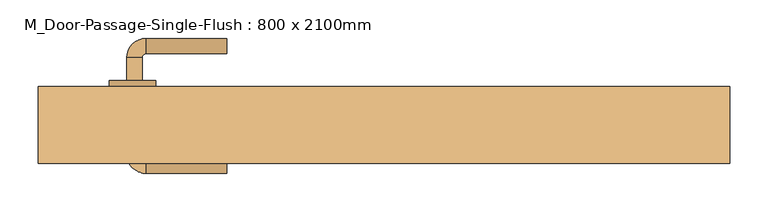
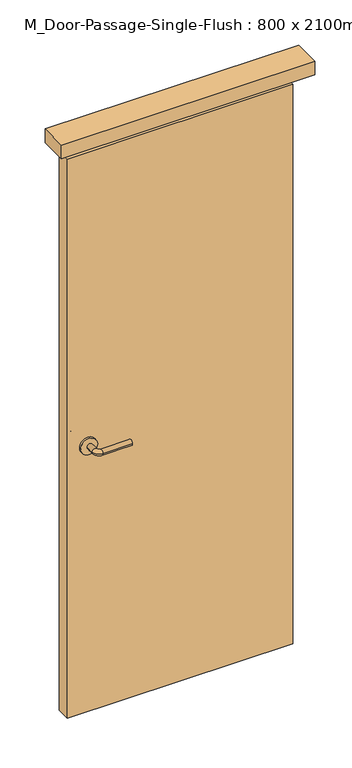
"""IFC4 building model written with IfcOpenShell, lengths in millimetres: door geometry, M_Door-Passage-Single-Flush : 800 x 2100mm."""

import ifcopenshell
import ifcopenshell.guid

model = None  # the IFC model being written
_history = None  # IfcOwnerHistory: only IFC2X3 demands one
_inside = {}  # id of a spatial element -> (the spatial element, [elements in it])
_under = {}  # id of a project, library or spatial element -> (it, [spatial elements below it])
_declared = {}  # id of a project -> (the project, [libraries it declares])
_typed = {}  # id of a type object -> (the type object, [elements of that type])
_made_of = {}  # id of a material, layer set ... -> (it, [elements and type objects made of it])


def new_model(schema):
    """Start an empty IFC model of exactly this schema.

    Asked for "IFC4X3", IfcOpenShell would pick the latest addendum, in which some entities
    have other attributes; the version numbers below select the first issue.
    IFC2X3 requires an IfcOwnerHistory on every rooted entity: one is made here for all.
    """
    global model, _history
    if schema == "IFC4X3":
        model = ifcopenshell.file(schema_version=(4, 3, 0, 0))
    else:
        model = ifcopenshell.file(schema=schema)
    _inside.clear()
    _under.clear()
    _declared.clear()
    _typed.clear()
    _made_of.clear()
    _history = None
    if model.schema == "IFC2X3":
        org = make("IfcOrganization", Name="unknown")
        user = make(
            "IfcPersonAndOrganization",
            ThePerson=make("IfcPerson", FamilyName="unknown"),
            TheOrganization=org,
        )
        app = make(
            "IfcApplication",
            ApplicationDeveloper=org,
            Version="unknown",
            ApplicationFullName="unknown",
            ApplicationIdentifier="unknown",
        )
        _history = make(
            "IfcOwnerHistory",
            OwningUser=user,
            OwningApplication=app,
            ChangeAction="ADDED",
            CreationDate=0,
        )
    return model


def make(cls, **values):
    """One entity of the class cls with the attributes given. An attribute that is None is left unset."""
    return model.create_entity(
        cls, **{name: value for name, value in values.items() if value is not None}
    )


def rooted(cls, **values):
    """An entity with a GlobalId (a new one), such as an element, a storey or a relation."""
    return make(cls, GlobalId=ifcopenshell.guid.new(), OwnerHistory=_history, **values)


def si_unit(unit_type, name, prefix=None):
    """IfcSIUnit, for example si_unit("LENGTHUNIT", "METRE", prefix="MILLI")."""
    return make("IfcSIUnit", UnitType=unit_type, Prefix=prefix, Name=name)


def assignment(units):
    """IfcUnitAssignment: the units of a project."""
    return None if units is None else make("IfcUnitAssignment", Units=units)


def point(xyz):
    """IfcCartesianPoint."""
    return None if xyz is None else make("IfcCartesianPoint", Coordinates=xyz)


def direction(xyz):
    """IfcDirection."""
    return None if xyz is None else make("IfcDirection", DirectionRatios=xyz)


def frame(location, z_axis=None, x_axis=None):
    """IfcAxis2Placement3D, a coordinate frame: its origin and axes. An axis left out is left unset."""
    return make(
        "IfcAxis2Placement3D",
        Location=point(location),
        Axis=direction(z_axis),
        RefDirection=direction(x_axis),
    )


def frame_2d(location, x_axis=None):
    """IfcAxis2Placement2D, a coordinate frame in the plane: its origin and x axis."""
    return make(
        "IfcAxis2Placement2D", Location=point(location), RefDirection=direction(x_axis)
    )


def origin():
    """The frame at (0, 0, 0) with its axes left unset."""
    return frame((0.0, 0.0, 0.0))


def origin_with_axes():
    """The frame at (0, 0, 0) with the z axis (0, 0, 1) and the x axis (1, 0, 0) written out."""
    return frame((0.0, 0.0, 0.0), z_axis=(0.0, 0.0, 1.0), x_axis=(1.0, 0.0, 0.0))


def place(relative_to, where):
    """IfcLocalPlacement: puts the frame where relative to a parent placement (None: the world)."""
    return make(
        "IfcLocalPlacement", PlacementRelTo=relative_to, RelativePlacement=where
    )


def context(
    kind, dimensions, precision=None, world=None, true_north=None, identifier=None
):
    """IfcGeometricRepresentationContext, for example the 3D "Model" context."""
    return make(
        "IfcGeometricRepresentationContext",
        ContextIdentifier=identifier,
        ContextType=kind,
        CoordinateSpaceDimension=dimensions,
        Precision=precision,
        WorldCoordinateSystem=world,
        TrueNorth=true_north,
    )


def project(units=None, contexts=None):
    """IfcProject with its units and contexts."""
    return rooted(
        "IfcProject",
        Name="project",
        RepresentationContexts=contexts,
        UnitsInContext=assignment(units),
    )


def spatial(cls, under=None, at=None, **own):
    """A site, building, storey or space (cls), placed at a placement, below another one or the project."""
    s = rooted(cls, ObjectPlacement=at, **own)
    if under is not None:
        _under.setdefault(under.id(), (under, []))[1].append(s)
    return s


def polyline(points):
    """IfcPolyline through the points."""
    return make("IfcPolyline", Points=[point(p) for p in points])


def circle_curve(where, radius):
    """IfcCircle in the frame where."""
    return make("IfcCircle", Position=where, Radius=radius)


def ellipse_curve(where, semi_axis1, semi_axis2):
    """IfcEllipse in the frame where."""
    return make(
        "IfcEllipse", Position=where, SemiAxis1=semi_axis1, SemiAxis2=semi_axis2
    )


def trimmed(basis, trim1, trim2, sense, master):
    """IfcTrimmedCurve: the piece of a basis curve between two trims."""
    return make(
        "IfcTrimmedCurve",
        BasisCurve=basis,
        Trim1=trim1,
        Trim2=trim2,
        SenseAgreement=sense,
        MasterRepresentation=master,
    )


def segment(curve, same_sense, transition):
    """IfcCompositeCurveSegment."""
    return make(
        "IfcCompositeCurveSegment",
        Transition=transition,
        SameSense=same_sense,
        ParentCurve=curve,
    )


def composite_curve(segments, self_intersect=None):
    """IfcCompositeCurve: segments joined end to end."""
    return make("IfcCompositeCurve", Segments=segments, SelfIntersect=self_intersect)


def outline(outer, holes=None, kind="AREA"):
    """IfcArbitraryClosedProfileDef: a profile drawn as a closed curve; with holes, ...WithVoids."""
    if holes is None:
        return make("IfcArbitraryClosedProfileDef", ProfileType=kind, OuterCurve=outer)
    return make(
        "IfcArbitraryProfileDefWithVoids",
        ProfileType=kind,
        OuterCurve=outer,
        InnerCurves=holes,
    )


def extrude(swept, where, along, depth):
    """IfcExtrudedAreaSolid: the profile swept, set in the frame where, extruded along a direction by depth."""
    return make(
        "IfcExtrudedAreaSolid",
        SweptArea=swept,
        Position=where,
        ExtrudedDirection=direction(along),
        Depth=depth,
    )


def shape(context_of_items, identifier, shape_type, items):
    """IfcShapeRepresentation: the items that make up one representation, for example the "Body"."""
    return make(
        "IfcShapeRepresentation",
        ContextOfItems=context_of_items,
        RepresentationIdentifier=identifier,
        RepresentationType=shape_type,
        Items=items,
    )


def source(mapping_origin, context_of_items, identifier, shape_type, items):
    """IfcRepresentationMap: a shape defined once, which mapped items show again and again."""
    return make(
        "IfcRepresentationMap",
        MappingOrigin=mapping_origin,
        MappedRepresentation=shape(context_of_items, identifier, shape_type, items),
    )


def transform(
    local_origin,
    x_axis=None,
    y_axis=None,
    z_axis=None,
    scale=None,
    scale2=None,
    scale3=None,
    uniform=True,
):
    """IfcCartesianTransformationOperator3D, or its non-uniform kind. x_axis, y_axis, z_axis: its Axis1, 2, 3."""
    if uniform:
        return make(
            "IfcCartesianTransformationOperator3D",
            Axis1=direction(x_axis),
            Axis2=direction(y_axis),
            LocalOrigin=point(local_origin),
            Scale=scale,
            Axis3=direction(z_axis),
        )
    return make(
        "IfcCartesianTransformationOperator3DnonUniform",
        Axis1=direction(x_axis),
        Axis2=direction(y_axis),
        LocalOrigin=point(local_origin),
        Scale=scale,
        Axis3=direction(z_axis),
        Scale2=scale2,
        Scale3=scale3,
    )


def mapped(mapping_source, mapping_target):
    """IfcMappedItem: shows the shape of a source again, moved by a transform."""
    return make(
        "IfcMappedItem", MappingSource=mapping_source, MappingTarget=mapping_target
    )


def made_of(thing, what):
    """Note that an element or type object is made of a material, layer set ...; save() writes the relation."""
    if what is not None:
        _made_of.setdefault(what.id(), (what, []))[1].append(thing)
    return thing


def element(
    cls,
    number,
    at=None,
    inside=None,
    cuts=None,
    type_object=None,
    material=None,
    context=None,
    identifier="Body",
    shape_type=None,
    held_by="IfcProductDefinitionShape",
    body=None,
    shapes=None,
    **own,
):
    """One element of the class cls, such as IfcWall. Its Tag is "e" and its number.

    at: its placement. inside: the storey or other place that contains it. cuts: it is an
    opening in that element (IfcRelVoidsElement). A single representation is given by context,
    identifier, shape_type and body (its items); several are given by shapes. held_by: the class
    of the entity that holds the representations. save() writes the other relations.
    """
    e = rooted(cls, Tag="e%d" % number, ObjectPlacement=at, **own)
    if body is not None:
        shapes = [shape(context, identifier, shape_type, body)]
    if shapes is not None:
        e.Representation = make(held_by, Representations=shapes)
    if inside is not None:
        _inside.setdefault(inside.id(), (inside, []))[1].append(e)
    if cuts is not None:
        rooted(
            "IfcRelVoidsElement", RelatingBuildingElement=cuts, RelatedOpeningElement=e
        )
    if type_object is not None:
        _typed.setdefault(type_object.id(), (type_object, []))[1].append(e)
    return made_of(e, material)


def aggregate(whole, parts):
    """IfcRelAggregates: a whole, such as a stair, and the parts it consists of."""
    return rooted("IfcRelAggregates", RelatingObject=whole, RelatedObjects=parts)


def save(model, path):
    """Write the relations noted so far, then the file.

    IfcRelAggregates (storeys below a building ...), IfcRelContainedInSpatialStructure (elements
    in a storey), IfcRelDefinesByType, IfcRelAssociatesMaterial and IfcRelDeclares: one each for
    every whole, place, type object, material and project.
    """
    for whole, parts in _under.values():
        aggregate(whole, parts)
    for where, things in _inside.values():
        rooted(
            "IfcRelContainedInSpatialStructure",
            RelatedElements=things,
            RelatingStructure=where,
        )
    for kind, things in _typed.values():
        rooted("IfcRelDefinesByType", RelatedObjects=things, RelatingType=kind)
    for what, things in _made_of.values():
        rooted("IfcRelAssociatesMaterial", RelatedObjects=things, RelatingMaterial=what)
    for by, libraries in _declared.values():
        rooted("IfcRelDeclares", RelatingContext=by, RelatedDefinitions=libraries)
    model.write(path)


def plane_surface(at):
    """IfcPlane: the flat surface through the origin of the frame at, square to its z axis."""
    return make("IfcPlane", Position=at)


def cylinder_surface(at, radius):
    """IfcCylindricalSurface: all points at the distance radius from the z axis of the frame at."""
    return make("IfcCylindricalSurface", Position=at, Radius=radius)


def revolved_surface(curve, axis_point, axis_direction):
    """IfcSurfaceOfRevolution: the curve turned about the line through axis_point along axis_direction."""
    return make(
        "IfcSurfaceOfRevolution",
        SweptCurve=make("IfcArbitraryOpenProfileDef", ProfileType="CURVE", Curve=curve),
        AxisPosition=make("IfcAxis1Placement", Location=point(axis_point), Axis=direction(axis_direction)),
    )


def advanced_brep(points, edges, surfaces, faces):
    """IfcAdvancedBrep: a solid bounded by faces that lie on surfaces and meet in shared edges.

    An edge is (start, end): straight between two places in points (the first is 0);
    or (start, end, curve); or (start, end, curve, False) where it runs against its curve.
    A face is (place in surfaces, loops), or (place, loops, False) where it looks against
    its surface's normal. A loop lists edges by number (the first is 1), with a minus sign
    where the edge is run from its end to its start. The first loop is the outer one.
    """
    corners = [point(p) for p in points]
    vertices = [make("IfcVertexPoint", VertexGeometry=c) for c in corners]
    made = []
    for start, end, *more in edges:
        made.append(
            make(
                "IfcEdgeCurve",
                EdgeStart=vertices[start],
                EdgeEnd=vertices[end],
                EdgeGeometry=more[0] if more else make("IfcPolyline", Points=[corners[start], corners[end]]),
                SameSense=more[1] if len(more) > 1 else True,
            )
        )
    hull = []
    for where, loops, *sense in faces:
        bounds = []
        for j, loop in enumerate(loops):
            ring = [make("IfcOrientedEdge", EdgeElement=made[abs(k) - 1], Orientation=k > 0) for k in loop]
            bounds.append(
                make(
                    "IfcFaceOuterBound" if j == 0 else "IfcFaceBound",
                    Bound=make("IfcEdgeLoop", EdgeList=ring),
                    Orientation=True,
                )
            )
        hull.append(make("IfcAdvancedFace", Bounds=bounds, FaceSurface=surfaces[where], SameSense=sense[0] if sense else True))
    return make("IfcAdvancedBrep", Outer=make("IfcClosedShell", CfsFaces=hull))


def m_door_passage_single_flush_800_x_2100mm_5f413de4(model_context):
    return source(origin(), model_context, "Body", "SolidModel", [
        advanced_brep(
        [(-334.990625, -1.65, 1000.0), (-314.990625, -1.65, 1000.0), (-314.990625, -31.65, 1000.0), (-334.990625, -31.65, 1000.0), (-309.990625, -36.65, 1000.0), (-309.990625, -56.65, 1000.0), (-204.990625, -56.65, 1000.0), (-204.990625, -36.65, 1000.0)],
        [
            (0, 1, circle_curve(frame((-324.990625, -1.65, 1000.0), z_axis=(0.0, 1.0, 0.0), x_axis=(1.0, 0.0, 0.0)), 10.0)),
            (1, 0, circle_curve(frame((-324.990625, -1.65, 1000.0), z_axis=(0.0, 1.0, 0.0), x_axis=(1.0, 0.0, 0.0)), 10.0)),
            (1, 2),
            (2, 3, circle_curve(frame((-324.990625, -31.65, 1000.0), z_axis=(0.0, 1.0, 0.0), x_axis=(1.0, 0.0, 0.0)), 10.0)),
            (3, 0),
            (3, 2, circle_curve(frame((-324.990625, -31.65, 1000.0), z_axis=(0.0, 1.0, 0.0), x_axis=(1.0, 0.0, 0.0)), 10.0)),
            (4, 5, circle_curve(frame((-309.990625, -46.65, 1000.0), z_axis=(-1.0, 0.0, 0.0), x_axis=(0.0, 1.0, 0.0)), 10.0)),
            (5, 3, circle_curve(frame((-309.990625, -31.65, 1000.0), z_axis=(0.0, 0.0, -1.0), x_axis=(-1.0, 0.0, 0.0)), 25.0)),
            (2, 4, circle_curve(frame((-309.990625, -31.65, 1000.0), z_axis=(0.0, 0.0, 1.0), x_axis=(-1.0, 0.0, 0.0)), 5.0)),
            (5, 4, circle_curve(frame((-309.990625, -46.65, 1000.0), z_axis=(-1.0, 0.0, 0.0), x_axis=(0.0, 1.0, 0.0)), 10.0)),
            (6, 7, circle_curve(frame((-204.990625, -46.65, 1000.0), z_axis=(1.0, 0.0, 0.0), x_axis=(0.0, 1.0, 0.0)), 10.0)),
            (7, 6, circle_curve(frame((-204.990625, -46.65, 1000.0), z_axis=(1.0, 0.0, 0.0), x_axis=(0.0, 1.0, 0.0)), 10.0)),
            (4, 7),
            (6, 5),
        ],
        [
            plane_surface(frame((-324.990625, -1.65, 1000.0), z_axis=(0.0, 1.0, 0.0), x_axis=(0.0, 0.0, 1.0))),
            cylinder_surface(frame((-324.990625, -1.65, 1000.0), z_axis=(0.0, 1.0, 0.0), x_axis=(1.0, 0.0, 0.0)), 10.0),
            revolved_surface(trimmed(ellipse_curve(frame((-324.990625, -31.65, 1000.0), z_axis=(0.0, -1.0, 0.0), x_axis=(1.0, 0.0, 0.0)), 10.0, 10.0), [point((-334.990625, -31.65, 1000.0))], [point((-314.990625, -31.65, 1000.0))], True, "CARTESIAN"), (-309.990625, -31.65, 1000.0), (0.0, 0.0, -1.0)),
            revolved_surface(trimmed(ellipse_curve(frame((-324.990625, -31.65, 1000.0), z_axis=(0.0, -1.0, 0.0), x_axis=(1.0, 0.0, 0.0)), 10.0, 10.0), [point((-314.990625, -31.65, 1000.0))], [point((-334.990625, -31.65, 1000.0))], True, "CARTESIAN"), (-309.990625, -31.65, 1000.0), (0.0, 0.0, -1.0)),
            plane_surface(frame((-204.990625, -46.65, 1000.0), z_axis=(1.0, 0.0, 0.0), x_axis=(0.0, 0.0, 1.0))),
            cylinder_surface(frame((-309.990625, -46.65, 1000.0), z_axis=(-1.0, 0.0, 0.0), x_axis=(0.0, 1.0, 0.0)), 10.0),
        ],
        [
            (0, [[1, 2]]),
            (1, [[3, 4, 5, -2]]),
            (1, [[-5, 6, -3, -1]]),
            (2, [[7, 8, -4, 9]]),
            (3, [[10, -9, -6, -8]]),
            (4, [[11, 12]]),
            (5, [[13, -11, 14, -7]]),
            (5, [[-14, -12, -13, -10]]),
        ],
    ),
        extrude(outline(composite_curve([segment(trimmed(circle_curve(frame_2d((1000.0, -327.490625)), 30.0), [point((1000.0, -357.490625))], [point((1000.0, -297.490625))], False, "CARTESIAN"), True, "CONTINUOUS"), segment(trimmed(circle_curve(frame_2d((1000.0, -327.490625)), 30.0), [point((1000.0, -297.490625))], [point((1000.0, -357.490625))], False, "CARTESIAN"), True, "CONTINUOUS")], self_intersect=False)), frame((0.0, -1.65, 0.0), z_axis=(0.0, 1.0, 0.0), x_axis=(0.0, 0.0, 1.0)), (0.0, 0.0, 1.0), 8.0),
        advanced_brep(
        [(-334.990625, 64.35, 1000.0), (-314.990625, 64.35, 1000.0), (-334.990625, 94.35, 1000.0), (-314.990625, 94.35, 1000.0), (-309.990625, 99.35, 1000.0), (-309.990625, 119.35, 1000.0), (-204.990625, 119.35, 1000.0), (-204.990625, 99.35, 1000.0)],
        [
            (0, 1, circle_curve(frame((-324.990625, 64.35, 1000.0), z_axis=(0.0, -1.0, 0.0), x_axis=(1.0, 0.0, 0.0)), 10.0)),
            (1, 0, circle_curve(frame((-324.990625, 64.35, 1000.0), z_axis=(0.0, -1.0, 0.0), x_axis=(1.0, 0.0, 0.0)), 10.0)),
            (0, 2),
            (2, 3, circle_curve(frame((-324.990625, 94.35, 1000.0), z_axis=(0.0, -1.0, 0.0), x_axis=(1.0, 0.0, 0.0)), 10.0)),
            (3, 1),
            (3, 2, circle_curve(frame((-324.990625, 94.35, 1000.0), z_axis=(0.0, -1.0, 0.0), x_axis=(1.0, 0.0, 0.0)), 10.0)),
            (4, 3, circle_curve(frame((-309.990625, 94.35, 1000.0), z_axis=(0.0, 0.0, 1.0), x_axis=(-1.0, 0.0, 0.0)), 5.0)),
            (2, 5, circle_curve(frame((-309.990625, 94.35, 1000.0), z_axis=(0.0, 0.0, -1.0), x_axis=(-1.0, 0.0, 0.0)), 25.0)),
            (5, 4, circle_curve(frame((-309.990625, 109.35, 1000.0), z_axis=(-1.0, 0.0, 0.0), x_axis=(0.0, -1.0, 0.0)), 10.0)),
            (4, 5, circle_curve(frame((-309.990625, 109.35, 1000.0), z_axis=(-1.0, 0.0, 0.0), x_axis=(0.0, -1.0, 0.0)), 10.0)),
            (6, 7, circle_curve(frame((-204.990625, 109.35, 1000.0), z_axis=(1.0, 0.0, 0.0), x_axis=(0.0, -1.0, 0.0)), 10.0)),
            (7, 6, circle_curve(frame((-204.990625, 109.35, 1000.0), z_axis=(1.0, 0.0, 0.0), x_axis=(0.0, -1.0, 0.0)), 10.0)),
            (5, 6),
            (7, 4),
        ],
        [
            plane_surface(frame((-324.990625, 64.35, 1000.0), z_axis=(0.0, -1.0, 0.0), x_axis=(0.0, 0.0, 1.0))),
            cylinder_surface(frame((-324.990625, 64.35, 1000.0), z_axis=(0.0, -1.0, 0.0), x_axis=(1.0, 0.0, 0.0)), 10.0),
            revolved_surface(trimmed(ellipse_curve(frame((-324.990625, 94.35, 1000.0), z_axis=(0.0, -1.0, 0.0), x_axis=(1.0, 0.0, 0.0)), 10.0, 10.0), [point((-334.990625, 94.35, 1000.0))], [point((-314.990625, 94.35, 1000.0))], True, "CARTESIAN"), (-309.990625, 94.35, 1000.0), (0.0, 0.0, -1.0)),
            revolved_surface(trimmed(ellipse_curve(frame((-324.990625, 94.35, 1000.0), z_axis=(0.0, -1.0, 0.0), x_axis=(1.0, 0.0, 0.0)), 10.0, 10.0), [point((-314.990625, 94.35, 1000.0))], [point((-334.990625, 94.35, 1000.0))], True, "CARTESIAN"), (-309.990625, 94.35, 1000.0), (0.0, 0.0, -1.0)),
            plane_surface(frame((-204.990625, 109.35, 1000.0), z_axis=(1.0, 0.0, 0.0), x_axis=(0.0, 0.0, 1.0))),
            cylinder_surface(frame((-309.990625, 109.35, 1000.0), z_axis=(-1.0, 0.0, 0.0), x_axis=(0.0, -1.0, 0.0)), 10.0),
        ],
        [
            (0, [[1, 2]]),
            (1, [[-1, 3, 4, 5]]),
            (1, [[-2, -5, 6, -3]]),
            (2, [[7, -4, 8, 9]]),
            (3, [[-8, -6, -7, 10]]),
            (4, [[11, 12]]),
            (5, [[-9, 13, -12, 14]]),
            (5, [[-10, -14, -11, -13]]),
        ],
    ),
        extrude(outline(composite_curve([segment(trimmed(circle_curve(frame_2d((1000.0, -327.490625)), 30.0), [point((1000.0, -357.490625))], [point((1000.0, -297.490625))], False, "CARTESIAN"), True, "CONTINUOUS"), segment(trimmed(circle_curve(frame_2d((1000.0, -327.490625)), 30.0), [point((1000.0, -297.490625))], [point((1000.0, -357.490625))], False, "CARTESIAN"), True, "CONTINUOUS")], self_intersect=False)), frame((0.0, 56.35, 0.0), z_axis=(0.0, 1.0, 0.0), x_axis=(0.0, 0.0, 1.0)), (0.0, 0.0, 1.0), 8.0),
        extrude(outline(polyline([(400.0, 6.35), (-400.0, 6.35), (-400.0, 56.35), (400.0, 56.35), (400.0, 6.35)])), origin_with_axes(), (0.0, 0.0, 1.0), 2100.0),
        extrude(outline(polyline([(450.0, 56.35), (450.0, -43.65), (-450.0, -43.65), (-450.0, 56.35), (450.0, 56.35)])), frame((0.0, 0.0, 2149.2), z_axis=(0.0, 0.0, 1.0), x_axis=(1.0, 0.0, 0.0)), (0.0, 0.0, 1.0), 50.8),
    ])


if __name__ == "__main__":
    model = new_model("IFC4")
    model_context = context("Model", 3, world=origin())
    ifc_project = project(units=[si_unit("LENGTHUNIT", "METRE", prefix="MILLI")], contexts=[model_context])
    site = spatial("IfcSite", under=ifc_project)
    building = spatial("IfcBuilding", under=site)
    placement = place(None, origin())
    m_door_passage_single_flush_800_x_2100mm_shape = m_door_passage_single_flush_800_x_2100mm_5f413de4(model_context)
    element("IfcDoor", 1, ObjectType="M_Door-Passage-Single-Flush : 800 x 2100mm", at=placement, inside=building, context=model_context, shape_type="MappedRepresentation", body=[
        mapped(m_door_passage_single_flush_800_x_2100mm_shape, transform((0.0, 0.0, 0.0), x_axis=(1.0, 0.0, 0.0), y_axis=(0.0, 1.0, 0.0), z_axis=(0.0, 0.0, 1.0))),
    ])
    save(model, "model.ifc")

# Revit data of these elements
# Type "M_Door-Passage-Single-Flush : 800 x 2100mm"
#   Type Mark = "46"
#   Assembly Code = "B2030200"
#   Analytic Construction = "Wooden"
#   Thickness = 50 mm
#   Thermal Resistance (R) = 0.455703 (m²·K)/W
#   Swing Angle [instance default] = 90.00°
#   Strike Height = 1000 mm
#   Rough Width [instance default] = 900 mm
#   Rough Height [instance default] = 2200 mm
#   MF Opening Height [instance default] = 100 mm
#   MF Opening Width [instance default] = 100 mm
#   Inset Calculate [instance default] = 105 mm
#   Masonry Inset [instance default] = 25 mm
#   Height = 2100 mm
#   Width = 800 mm
#   Heat Transfer Coefficient (U) = 2.19465 W/(m²·K)
#   Masonry Frame Depth = 100 mm
#   Masonry Frame [instance default] = yes
#   Function = 1
#   Dry Wall Frame [instance default] = no
#   Panel Material = Wood - Birch
#   Frame Material = Metal - Paint Finish - Grey
#   Door Handle Material = Aluminum
#   Visual Light Transmittance = 0
#   Solar Heat Gain Coefficient = 0
#   Wall Closure = (empty or 0)
# Element 1 (IfcDoor, "M_Door-Passage-Single-Flush : 800 x 2100mm")
#   Materials on its faces: "Aluminum", "Wood - Birch", "Metal - Paint Finish - Grey"
# Materials
#   "Wood - Birch": class "Wood", colour RGB 173 132 96, transparency 0, Cost = 0
#   "Metal - Paint Finish - Grey": class "Paint", colour RGB 178 178 178, transparency 0, Cost = 0
#   "Aluminum": class "Metal", colour RGB 244 245 246, transparency 0, Description = "Aluminum 6061", Cost = 0
